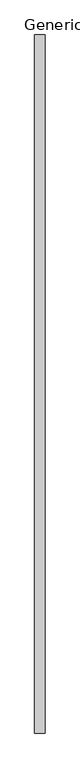
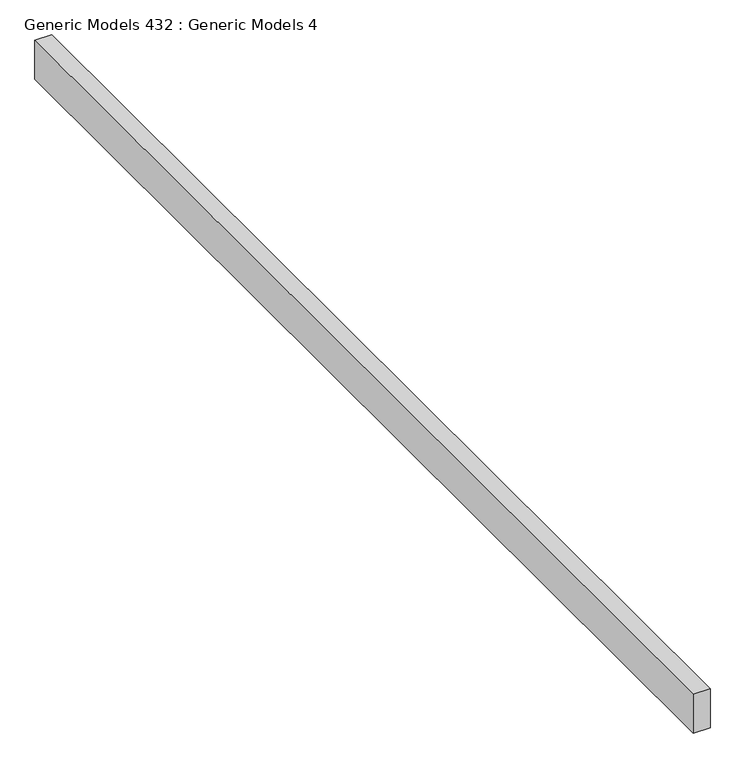
"""IFC4 building model written with IfcOpenShell, lengths in millimetres: proxy geometry, Generic Models 432 : Generic Models 4."""

import ifcopenshell
import ifcopenshell.guid

model = None  # the IFC model being written
_history = None  # IfcOwnerHistory: only IFC2X3 demands one
_inside = {}  # id of a spatial element -> (the spatial element, [elements in it])
_under = {}  # id of a project, library or spatial element -> (it, [spatial elements below it])
_declared = {}  # id of a project -> (the project, [libraries it declares])
_typed = {}  # id of a type object -> (the type object, [elements of that type])
_made_of = {}  # id of a material, layer set ... -> (it, [elements and type objects made of it])


def new_model(schema):
    """Start an empty IFC model of exactly this schema.

    Asked for "IFC4X3", IfcOpenShell would pick the latest addendum, in which some entities
    have other attributes; the version numbers below select the first issue.
    IFC2X3 requires an IfcOwnerHistory on every rooted entity: one is made here for all.
    """
    global model, _history
    if schema == "IFC4X3":
        model = ifcopenshell.file(schema_version=(4, 3, 0, 0))
    else:
        model = ifcopenshell.file(schema=schema)
    _inside.clear()
    _under.clear()
    _declared.clear()
    _typed.clear()
    _made_of.clear()
    _history = None
    if model.schema == "IFC2X3":
        org = make("IfcOrganization", Name="unknown")
        user = make(
            "IfcPersonAndOrganization",
            ThePerson=make("IfcPerson", FamilyName="unknown"),
            TheOrganization=org,
        )
        app = make(
            "IfcApplication",
            ApplicationDeveloper=org,
            Version="unknown",
            ApplicationFullName="unknown",
            ApplicationIdentifier="unknown",
        )
        _history = make(
            "IfcOwnerHistory",
            OwningUser=user,
            OwningApplication=app,
            ChangeAction="ADDED",
            CreationDate=0,
        )
    return model


def make(cls, **values):
    """One entity of the class cls with the attributes given. An attribute that is None is left unset."""
    return model.create_entity(
        cls, **{name: value for name, value in values.items() if value is not None}
    )


def rooted(cls, **values):
    """An entity with a GlobalId (a new one), such as an element, a storey or a relation."""
    return make(cls, GlobalId=ifcopenshell.guid.new(), OwnerHistory=_history, **values)


def si_unit(unit_type, name, prefix=None):
    """IfcSIUnit, for example si_unit("LENGTHUNIT", "METRE", prefix="MILLI")."""
    return make("IfcSIUnit", UnitType=unit_type, Prefix=prefix, Name=name)


def assignment(units):
    """IfcUnitAssignment: the units of a project."""
    return None if units is None else make("IfcUnitAssignment", Units=units)


def point(xyz):
    """IfcCartesianPoint."""
    return None if xyz is None else make("IfcCartesianPoint", Coordinates=xyz)


def direction(xyz):
    """IfcDirection."""
    return None if xyz is None else make("IfcDirection", DirectionRatios=xyz)


def frame(location, z_axis=None, x_axis=None):
    """IfcAxis2Placement3D, a coordinate frame: its origin and axes. An axis left out is left unset."""
    return make(
        "IfcAxis2Placement3D",
        Location=point(location),
        Axis=direction(z_axis),
        RefDirection=direction(x_axis),
    )


def origin():
    """The frame at (0, 0, 0) with its axes left unset."""
    return frame((0.0, 0.0, 0.0))


def place(relative_to, where):
    """IfcLocalPlacement: puts the frame where relative to a parent placement (None: the world)."""
    return make(
        "IfcLocalPlacement", PlacementRelTo=relative_to, RelativePlacement=where
    )


def context(
    kind, dimensions, precision=None, world=None, true_north=None, identifier=None
):
    """IfcGeometricRepresentationContext, for example the 3D "Model" context."""
    return make(
        "IfcGeometricRepresentationContext",
        ContextIdentifier=identifier,
        ContextType=kind,
        CoordinateSpaceDimension=dimensions,
        Precision=precision,
        WorldCoordinateSystem=world,
        TrueNorth=true_north,
    )


def project(units=None, contexts=None):
    """IfcProject with its units and contexts."""
    return rooted(
        "IfcProject",
        Name="project",
        RepresentationContexts=contexts,
        UnitsInContext=assignment(units),
    )


def spatial(cls, under=None, at=None, **own):
    """A site, building, storey or space (cls), placed at a placement, below another one or the project."""
    s = rooted(cls, ObjectPlacement=at, **own)
    if under is not None:
        _under.setdefault(under.id(), (under, []))[1].append(s)
    return s


def polyline(points):
    """IfcPolyline through the points."""
    return make("IfcPolyline", Points=[point(p) for p in points])


def outline(outer, holes=None, kind="AREA"):
    """IfcArbitraryClosedProfileDef: a profile drawn as a closed curve; with holes, ...WithVoids."""
    if holes is None:
        return make("IfcArbitraryClosedProfileDef", ProfileType=kind, OuterCurve=outer)
    return make(
        "IfcArbitraryProfileDefWithVoids",
        ProfileType=kind,
        OuterCurve=outer,
        InnerCurves=holes,
    )


def extrude(swept, where, along, depth):
    """IfcExtrudedAreaSolid: the profile swept, set in the frame where, extruded along a direction by depth."""
    return make(
        "IfcExtrudedAreaSolid",
        SweptArea=swept,
        Position=where,
        ExtrudedDirection=direction(along),
        Depth=depth,
    )


def shape(context_of_items, identifier, shape_type, items):
    """IfcShapeRepresentation: the items that make up one representation, for example the "Body"."""
    return make(
        "IfcShapeRepresentation",
        ContextOfItems=context_of_items,
        RepresentationIdentifier=identifier,
        RepresentationType=shape_type,
        Items=items,
    )


def source(mapping_origin, context_of_items, identifier, shape_type, items):
    """IfcRepresentationMap: a shape defined once, which mapped items show again and again."""
    return make(
        "IfcRepresentationMap",
        MappingOrigin=mapping_origin,
        MappedRepresentation=shape(context_of_items, identifier, shape_type, items),
    )


def transform(
    local_origin,
    x_axis=None,
    y_axis=None,
    z_axis=None,
    scale=None,
    scale2=None,
    scale3=None,
    uniform=True,
):
    """IfcCartesianTransformationOperator3D, or its non-uniform kind. x_axis, y_axis, z_axis: its Axis1, 2, 3."""
    if uniform:
        return make(
            "IfcCartesianTransformationOperator3D",
            Axis1=direction(x_axis),
            Axis2=direction(y_axis),
            LocalOrigin=point(local_origin),
            Scale=scale,
            Axis3=direction(z_axis),
        )
    return make(
        "IfcCartesianTransformationOperator3DnonUniform",
        Axis1=direction(x_axis),
        Axis2=direction(y_axis),
        LocalOrigin=point(local_origin),
        Scale=scale,
        Axis3=direction(z_axis),
        Scale2=scale2,
        Scale3=scale3,
    )


def mapped(mapping_source, mapping_target):
    """IfcMappedItem: shows the shape of a source again, moved by a transform."""
    return make(
        "IfcMappedItem", MappingSource=mapping_source, MappingTarget=mapping_target
    )


def made_of(thing, what):
    """Note that an element or type object is made of a material, layer set ...; save() writes the relation."""
    if what is not None:
        _made_of.setdefault(what.id(), (what, []))[1].append(thing)
    return thing


def element(
    cls,
    number,
    at=None,
    inside=None,
    cuts=None,
    type_object=None,
    material=None,
    context=None,
    identifier="Body",
    shape_type=None,
    held_by="IfcProductDefinitionShape",
    body=None,
    shapes=None,
    **own,
):
    """One element of the class cls, such as IfcWall. Its Tag is "e" and its number.

    at: its placement. inside: the storey or other place that contains it. cuts: it is an
    opening in that element (IfcRelVoidsElement). A single representation is given by context,
    identifier, shape_type and body (its items); several are given by shapes. held_by: the class
    of the entity that holds the representations. save() writes the other relations.
    """
    e = rooted(cls, Tag="e%d" % number, ObjectPlacement=at, **own)
    if body is not None:
        shapes = [shape(context, identifier, shape_type, body)]
    if shapes is not None:
        e.Representation = make(held_by, Representations=shapes)
    if inside is not None:
        _inside.setdefault(inside.id(), (inside, []))[1].append(e)
    if cuts is not None:
        rooted(
            "IfcRelVoidsElement", RelatingBuildingElement=cuts, RelatedOpeningElement=e
        )
    if type_object is not None:
        _typed.setdefault(type_object.id(), (type_object, []))[1].append(e)
    return made_of(e, material)


def aggregate(whole, parts):
    """IfcRelAggregates: a whole, such as a stair, and the parts it consists of."""
    return rooted("IfcRelAggregates", RelatingObject=whole, RelatedObjects=parts)


def save(model, path):
    """Write the relations noted so far, then the file.

    IfcRelAggregates (storeys below a building ...), IfcRelContainedInSpatialStructure (elements
    in a storey), IfcRelDefinesByType, IfcRelAssociatesMaterial and IfcRelDeclares: one each for
    every whole, place, type object, material and project.
    """
    for whole, parts in _under.values():
        aggregate(whole, parts)
    for where, things in _inside.values():
        rooted(
            "IfcRelContainedInSpatialStructure",
            RelatedElements=things,
            RelatingStructure=where,
        )
    for kind, things in _typed.values():
        rooted("IfcRelDefinesByType", RelatedObjects=things, RelatingType=kind)
    for what, things in _made_of.values():
        rooted("IfcRelAssociatesMaterial", RelatedObjects=things, RelatingMaterial=what)
    for by, libraries in _declared.values():
        rooted("IfcRelDeclares", RelatingContext=by, RelatedDefinitions=libraries)
    model.write(path)


def generic_models_432_generic_models_4_22d0f852(model_context):
    return source(origin(), model_context, "Body", "SweptSolid", [
        extrude(outline(polyline([(8553.2763705, -6864.9230338), (8486.3473704, -6864.9230338), (8486.3473704, -2343.7230338), (8553.2763704, -2343.7230338), (8553.2763705, -6864.9230338)])), frame((0.0, 0.0, 126383.796), z_axis=(0.0, 0.0, 1.0), x_axis=(1.0, 0.0, 0.0)), (0.0, 0.0, 1.0), 162.0790924),
    ])


if __name__ == "__main__":
    model = new_model("IFC4")
    model_context = context("Model", 3, world=origin())
    ifc_project = project(units=[si_unit("LENGTHUNIT", "METRE", prefix="MILLI")], contexts=[model_context])
    site = spatial("IfcSite", under=ifc_project)
    building = spatial("IfcBuilding", under=site)
    placement = place(None, origin())
    generic_models_432_generic_models_4_shape = generic_models_432_generic_models_4_22d0f852(model_context)
    element("IfcBuildingElementProxy", 1, Name="Generic Models 432 : Generic Models 4", ObjectType="Generic Models 432 : Generic Models 4", at=placement, inside=building, context=model_context, shape_type="MappedRepresentation", body=[
        mapped(generic_models_432_generic_models_4_shape, transform((0.0, 0.0, 0.0), x_axis=(1.0, 0.0, 0.0), y_axis=(0.0, 1.0, 0.0), z_axis=(0.0, 0.0, 1.0))),
    ])
    save(model, "model.ifc")

# Revit data of these elements
# Element 1 (IfcBuildingElementProxy, "Generic Models 432 : Generic Models 4")
#   Materials on its faces: "_2X BLOCKING AS REQUIRED"
# Materials
#   "_2X BLOCKING AS REQUIRED": class "Generic", colour RGB 177 130 114, transparency 0, Cost = 0
